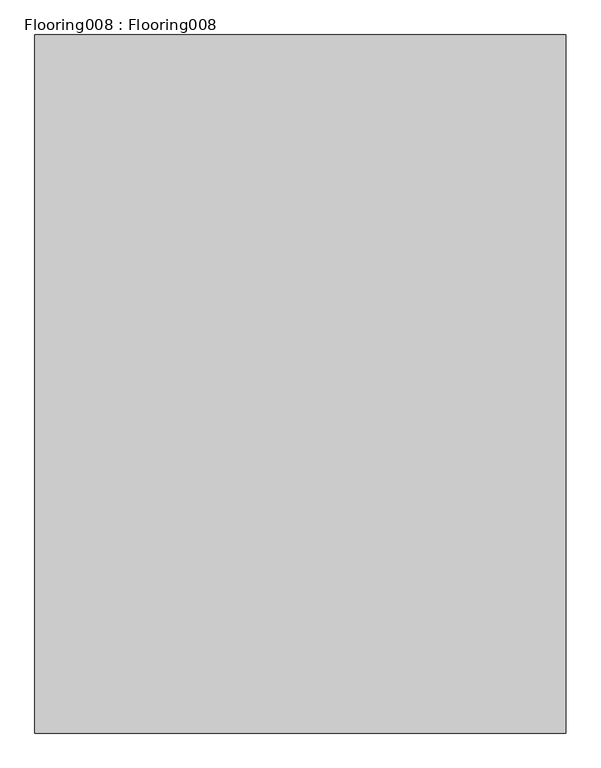
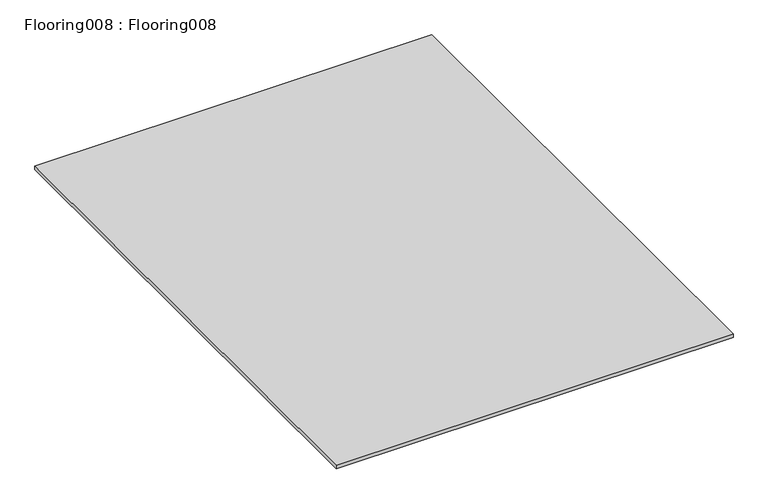
"""IFC4 building model written with IfcOpenShell, lengths in millimetres: proxy geometry, Flooring008 : Flooring008."""

from ifc_helpers import new_model, si_unit, frame, origin, place, context, project, spatial, polyline, outline, extrude, source, transform, mapped, element, save


def flooring008_flooring008_03dc8a51(model_context):
    return source(origin(), model_context, "Body", "SweptSolid", [
        extrude(outline(polyline([(3694.5383192, 7649.8526877), (3694.5383192, 10278.0250834), (5694.5383192, 10278.0250834), (5694.5383192, 7649.8526877), (3694.5383192, 7649.8526877)])), frame((0.0, 0.0, 40138.0976562), z_axis=(0.0, 0.0, 1.0), x_axis=(1.0, 0.0, 0.0)), (0.0, 0.0, 1.0), 19.05),
    ])


if __name__ == "__main__":
    model = new_model("IFC4")
    model_context = context("Model", 3, world=origin())
    ifc_project = project(units=[si_unit("LENGTHUNIT", "METRE", prefix="MILLI")], contexts=[model_context])
    site = spatial("IfcSite", under=ifc_project)
    building = spatial("IfcBuilding", under=site)
    placement = place(None, origin())
    flooring008_flooring008_shape = flooring008_flooring008_03dc8a51(model_context)
    element("IfcBuildingElementProxy", 1, Name="Flooring008 : Flooring008", ObjectType="Flooring008 : Flooring008", at=placement, inside=building, context=model_context, shape_type="MappedRepresentation", body=[
        mapped(flooring008_flooring008_shape, transform((0.0, 0.0, 0.0), x_axis=(1.0, 0.0, 0.0), y_axis=(0.0, 1.0, 0.0), z_axis=(0.0, 0.0, 1.0))),
    ])
    save(model, "model.ifc")

# Revit data of these elements
# Type "Flooring008 : Flooring008"
#   NameOverride = "Flooring008"
# Element 1 (IfcBuildingElementProxy, "Flooring008 : Flooring008")
#   Materials on its faces: "WOOD FLOORING (SPEC TBD)"
# Materials
#   "WOOD FLOORING (SPEC TBD)": class "Unassigned", colour RGB 201 162 125, transparency 0
